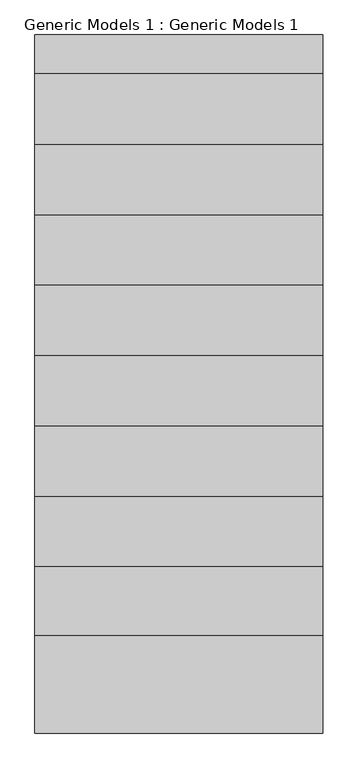
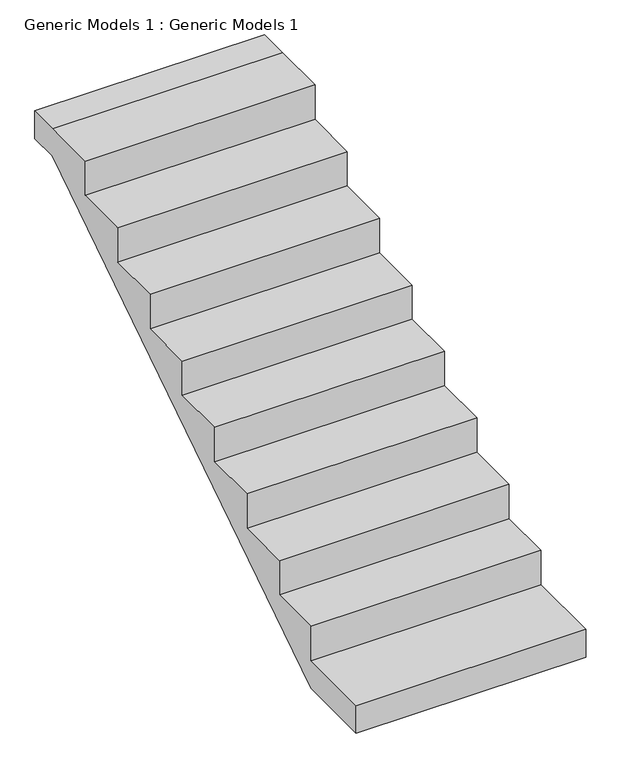
"""IFC4 building model written with IfcOpenShell, lengths in millimetres: proxy geometry, Generic Models 1 : Generic Models 1."""

from ifc_helpers import new_model, si_unit, frame, origin, place, context, project, spatial, polyline, outline, extrude, source, transform, mapped, element, save


def generic_models_1_generic_models_1_c3b3df0b(model_context):
    return source(origin(), model_context, "Body", "SweptSolid", [
        extrude(outline(polyline([(23365.484552, 1575.0), (23630.484552, 1575.0), (23630.484552, 1750.0), (23900.484552, 1750.0), (23900.484552, 1925.0), (24170.484552, 1925.0), (24170.484552, 2100.0), (24440.484552, 2100.0), (24440.484552, 2273.0), (24710.484552, 2273.0), (24710.484552, 2450.0), (24980.484552, 2450.0), (24980.484552, 2625.0), (25250.484552, 2625.0), (25250.484552, 2800.0), (25520.484552, 2800.0), (25670.484552, 2800.0), (25670.484552, 2660.0), (25525.484552, 2660.0), (23365.484552, 1260.0), (22990.484552, 1260.0), (22990.484552, 1400.0), (23365.484552, 1400.0), (23365.484552, 1575.0)])), frame((81451.2978475, 0.0, 0.0), z_axis=(1.0, 0.0, 0.0), x_axis=(0.0, 1.0, 0.0)), (0.0, 0.0, 1.0), 1105.7161874),
    ])


if __name__ == "__main__":
    model = new_model("IFC4")
    model_context = context("Model", 3, world=origin())
    ifc_project = project(units=[si_unit("LENGTHUNIT", "METRE", prefix="MILLI")], contexts=[model_context])
    site = spatial("IfcSite", under=ifc_project)
    building = spatial("IfcBuilding", under=site)
    placement = place(None, origin())
    generic_models_1_generic_models_1_shape = generic_models_1_generic_models_1_c3b3df0b(model_context)
    element("IfcBuildingElementProxy", 1, Name="Generic Models 1 : Generic Models 1", ObjectType="Generic Models 1 : Generic Models 1", at=placement, inside=building, context=model_context, shape_type="MappedRepresentation", body=[
        mapped(generic_models_1_generic_models_1_shape, transform((0.0, 0.0, 0.0), x_axis=(1.0, 0.0, 0.0), y_axis=(0.0, 1.0, 0.0), z_axis=(0.0, 0.0, 1.0))),
    ])
    save(model, "model.ifc")

# Revit data of these elements
# Type "Generic Models 1 : Generic Models 1"
#   Type Mark = "Prefab_staircase"
